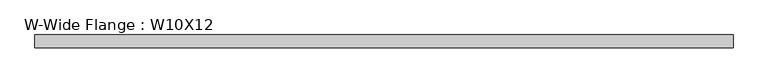
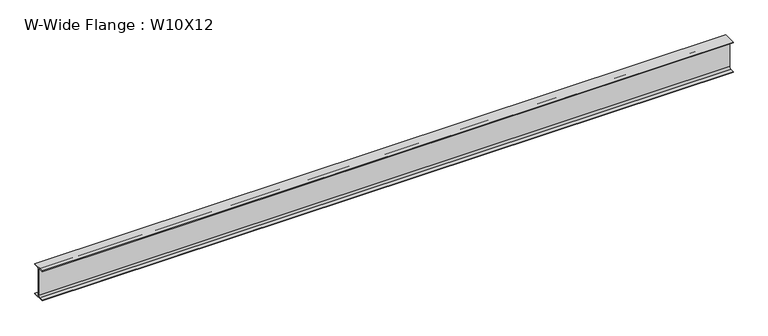
"""IFC4 building model written with IfcOpenShell, lengths in millimetres: beam geometry, W-Wide Flange : W10X12."""

from ifc_helpers import new_model, si_unit, point, frame, frame_2d, origin, place, context, project, spatial, polyline, circle_curve, trimmed, segment, composite_curve, outline, extrude, source, transform, mapped, element, save


def w_wide_flange_w10x12_049afd95(model_context):
    return source(origin(), model_context, "Body", "SweptSolid", [
        extrude(outline(composite_curve([segment(polyline([(50.292, -120.015), (50.292, -125.349), (-50.292, -125.349), (-50.292, -120.015), (-16.129, -120.015)]), True, "CONTINUOUS"), segment(trimmed(circle_curve(frame_2d((-16.129, -106.299)), 13.716), [point((-16.129, -120.015))], [point((-2.413, -106.299))], True, "CARTESIAN"), True, "CONTINUOUS"), segment(polyline([(-2.413, -106.299), (-2.413, 106.299)]), True, "CONTINUOUS"), segment(trimmed(circle_curve(frame_2d((-16.129, 106.299)), 13.716), [point((-2.413, 106.299))], [point((-16.129, 120.015))], True, "CARTESIAN"), True, "CONTINUOUS"), segment(polyline([(-16.129, 120.015), (-50.292, 120.015), (-50.292, 125.349), (50.292, 125.349), (50.292, 120.015), (16.129, 120.015)]), True, "CONTINUOUS"), segment(trimmed(circle_curve(frame_2d((16.129, 106.299)), 13.716), [point((16.129, 120.015))], [point((2.413, 106.299))], True, "CARTESIAN"), True, "CONTINUOUS"), segment(polyline([(2.413, 106.299), (2.413, -106.299)]), True, "CONTINUOUS"), segment(trimmed(circle_curve(frame_2d((16.129, -106.299)), 13.716), [point((2.413, -106.299))], [point((16.129, -120.015))], True, "CARTESIAN"), True, "CONTINUOUS"), segment(polyline([(16.129, -120.015), (50.292, -120.015)]), True, "CONTINUOUS")], self_intersect=False)), frame((-2731.8335, 0.0, 0.0), z_axis=(1.0, 0.0, 0.0), x_axis=(0.0, 1.0, 0.0)), (0.0, 0.0, 1.0), 5463.667),
    ])


if __name__ == "__main__":
    model = new_model("IFC4")
    model_context = context("Model", 3, world=origin())
    ifc_project = project(units=[si_unit("LENGTHUNIT", "METRE", prefix="MILLI")], contexts=[model_context])
    site = spatial("IfcSite", under=ifc_project)
    building = spatial("IfcBuilding", under=site)
    placement = place(None, origin())
    w_wide_flange_w10x12_shape = w_wide_flange_w10x12_049afd95(model_context)
    element("IfcBeam", 1, ObjectType="W-Wide Flange : W10X12", at=placement, inside=building, context=model_context, shape_type="MappedRepresentation", body=[
        mapped(w_wide_flange_w10x12_shape, transform((0.0, 0.0, 0.0), x_axis=(1.0, 0.0, 0.0), y_axis=(0.0, 1.0, 0.0), z_axis=(0.0, 0.0, 1.0))),
    ])
    save(model, "model.ifc")

# Revit data of these elements
# Type "W-Wide Flange : W10X12"
#   Assembly Code = "B10"
#   W = 12
#   Length [instance default] = 1524 mm
#   bf = 100.584 mm
#   d = 250.698 mm
#   k = 19.05 mm
#   k2 = 13.716 mm
#   tf = 5.334 mm
#   tw = 4.826 mm
#   A = 0.00228387 m²
#   Structural Material [instance default] = Steel ASTM A992
# Element 1 (IfcBeam, "W-Wide Flange : W10X12")
#   Structural Material = Aluminum, Anodized Red
#   Materials on its faces: "Aluminum, Anodized Red"
# Materials
#   "Steel ASTM A992": class "Metal", colour RGB 128 0 0, transparency 0, Description = "Structural steel 50ksi", Cost = 0
#   "Aluminum, Anodized Red": class "Metal", colour RGB 120 120 120, transparency 0, Description = "Anodized aluminum, red", Cost = 0
